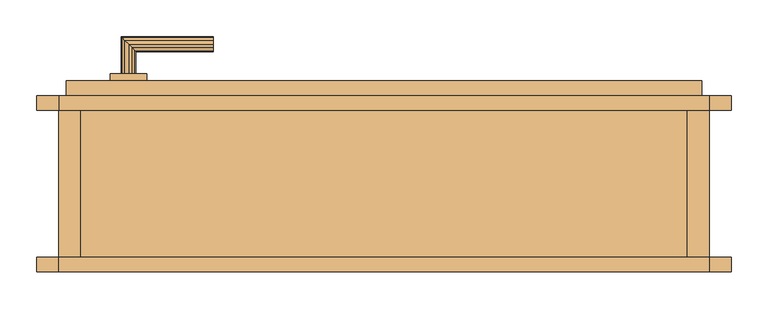
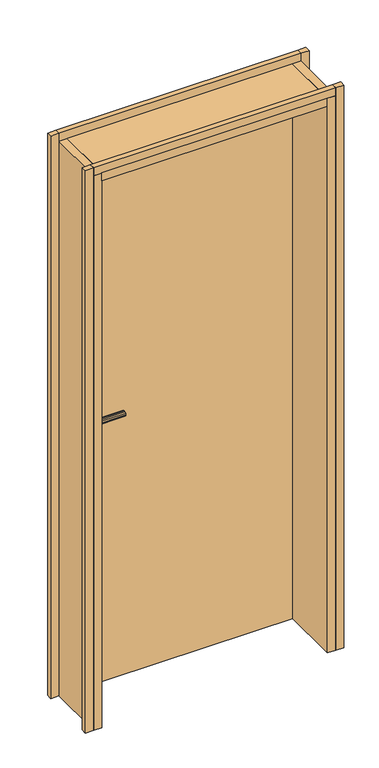
"""IFC4 building model written with IfcOpenShell, lengths in millimetres: door geometry, Tür."""

import ifcopenshell
import ifcopenshell.guid

model = None  # the IFC model being written
_history = None  # IfcOwnerHistory: only IFC2X3 demands one
_inside = {}  # id of a spatial element -> (the spatial element, [elements in it])
_under = {}  # id of a project, library or spatial element -> (it, [spatial elements below it])
_declared = {}  # id of a project -> (the project, [libraries it declares])
_typed = {}  # id of a type object -> (the type object, [elements of that type])
_made_of = {}  # id of a material, layer set ... -> (it, [elements and type objects made of it])


def new_model(schema):
    """Start an empty IFC model of exactly this schema.

    Asked for "IFC4X3", IfcOpenShell would pick the latest addendum, in which some entities
    have other attributes; the version numbers below select the first issue.
    IFC2X3 requires an IfcOwnerHistory on every rooted entity: one is made here for all.
    """
    global model, _history
    if schema == "IFC4X3":
        model = ifcopenshell.file(schema_version=(4, 3, 0, 0))
    else:
        model = ifcopenshell.file(schema=schema)
    _inside.clear()
    _under.clear()
    _declared.clear()
    _typed.clear()
    _made_of.clear()
    _history = None
    if model.schema == "IFC2X3":
        org = make("IfcOrganization", Name="unknown")
        user = make(
            "IfcPersonAndOrganization",
            ThePerson=make("IfcPerson", FamilyName="unknown"),
            TheOrganization=org,
        )
        app = make(
            "IfcApplication",
            ApplicationDeveloper=org,
            Version="unknown",
            ApplicationFullName="unknown",
            ApplicationIdentifier="unknown",
        )
        _history = make(
            "IfcOwnerHistory",
            OwningUser=user,
            OwningApplication=app,
            ChangeAction="ADDED",
            CreationDate=0,
        )
    return model


def make(cls, **values):
    """One entity of the class cls with the attributes given. An attribute that is None is left unset."""
    return model.create_entity(
        cls, **{name: value for name, value in values.items() if value is not None}
    )


def rooted(cls, **values):
    """An entity with a GlobalId (a new one), such as an element, a storey or a relation."""
    return make(cls, GlobalId=ifcopenshell.guid.new(), OwnerHistory=_history, **values)


def si_unit(unit_type, name, prefix=None):
    """IfcSIUnit, for example si_unit("LENGTHUNIT", "METRE", prefix="MILLI")."""
    return make("IfcSIUnit", UnitType=unit_type, Prefix=prefix, Name=name)


def assignment(units):
    """IfcUnitAssignment: the units of a project."""
    return None if units is None else make("IfcUnitAssignment", Units=units)


def point(xyz):
    """IfcCartesianPoint."""
    return None if xyz is None else make("IfcCartesianPoint", Coordinates=xyz)


def direction(xyz):
    """IfcDirection."""
    return None if xyz is None else make("IfcDirection", DirectionRatios=xyz)


def frame(location, z_axis=None, x_axis=None):
    """IfcAxis2Placement3D, a coordinate frame: its origin and axes. An axis left out is left unset."""
    return make(
        "IfcAxis2Placement3D",
        Location=point(location),
        Axis=direction(z_axis),
        RefDirection=direction(x_axis),
    )


def origin():
    """The frame at (0, 0, 0) with its axes left unset."""
    return frame((0.0, 0.0, 0.0))


def place(relative_to, where):
    """IfcLocalPlacement: puts the frame where relative to a parent placement (None: the world)."""
    return make(
        "IfcLocalPlacement", PlacementRelTo=relative_to, RelativePlacement=where
    )


def context(
    kind, dimensions, precision=None, world=None, true_north=None, identifier=None
):
    """IfcGeometricRepresentationContext, for example the 3D "Model" context."""
    return make(
        "IfcGeometricRepresentationContext",
        ContextIdentifier=identifier,
        ContextType=kind,
        CoordinateSpaceDimension=dimensions,
        Precision=precision,
        WorldCoordinateSystem=world,
        TrueNorth=true_north,
    )


def project(units=None, contexts=None):
    """IfcProject with its units and contexts."""
    return rooted(
        "IfcProject",
        Name="project",
        RepresentationContexts=contexts,
        UnitsInContext=assignment(units),
    )


def spatial(cls, under=None, at=None, **own):
    """A site, building, storey or space (cls), placed at a placement, below another one or the project."""
    s = rooted(cls, ObjectPlacement=at, **own)
    if under is not None:
        _under.setdefault(under.id(), (under, []))[1].append(s)
    return s


def polyline(points):
    """IfcPolyline through the points."""
    return make("IfcPolyline", Points=[point(p) for p in points])


def outline(outer, holes=None, kind="AREA"):
    """IfcArbitraryClosedProfileDef: a profile drawn as a closed curve; with holes, ...WithVoids."""
    if holes is None:
        return make("IfcArbitraryClosedProfileDef", ProfileType=kind, OuterCurve=outer)
    return make(
        "IfcArbitraryProfileDefWithVoids",
        ProfileType=kind,
        OuterCurve=outer,
        InnerCurves=holes,
    )


def extrude(swept, where, along, depth):
    """IfcExtrudedAreaSolid: the profile swept, set in the frame where, extruded along a direction by depth."""
    return make(
        "IfcExtrudedAreaSolid",
        SweptArea=swept,
        Position=where,
        ExtrudedDirection=direction(along),
        Depth=depth,
    )


def faces_of(points, faces, orient=None, outer=None):
    """IfcFace entities. A face is a list of loops; a loop is a list of indices into points, from 0.

    orient and outer hold one flag for each loop. By default every Orientation is true, the
    first loop of a face is its IfcFaceOuterBound and the others are IfcFaceBound.
    """
    made = []
    for i, loops in enumerate(faces):
        bounds = []
        for j, loop in enumerate(loops):
            is_outer = j == 0 if outer is None else outer[i][j]
            bounds.append(
                make(
                    "IfcFaceOuterBound" if is_outer else "IfcFaceBound",
                    Bound=make("IfcPolyLoop", Polygon=[points[k] for k in loop]),
                    Orientation=True if orient is None else orient[i][j],
                )
            )
        made.append(make("IfcFace", Bounds=bounds))
    return made


def faceted_brep(points, faces, orient=None, outer=None, voids=None):
    """IfcFacetedBrep: a solid bounded by flat faces; with voids (closed shells), ...WithVoids."""
    shared = [point(p) for p in points]
    hull = make("IfcClosedShell", CfsFaces=faces_of(shared, faces, orient, outer))
    if voids is None:
        return make("IfcFacetedBrep", Outer=hull)
    return make(
        "IfcFacetedBrepWithVoids",
        Outer=hull,
        Voids=[
            make(cls, CfsFaces=faces_of(shared, fs, o, b)) for cls, fs, o, b in voids
        ],
    )


def shape(context_of_items, identifier, shape_type, items):
    """IfcShapeRepresentation: the items that make up one representation, for example the "Body"."""
    return make(
        "IfcShapeRepresentation",
        ContextOfItems=context_of_items,
        RepresentationIdentifier=identifier,
        RepresentationType=shape_type,
        Items=items,
    )


def source(mapping_origin, context_of_items, identifier, shape_type, items):
    """IfcRepresentationMap: a shape defined once, which mapped items show again and again."""
    return make(
        "IfcRepresentationMap",
        MappingOrigin=mapping_origin,
        MappedRepresentation=shape(context_of_items, identifier, shape_type, items),
    )


def transform(
    local_origin,
    x_axis=None,
    y_axis=None,
    z_axis=None,
    scale=None,
    scale2=None,
    scale3=None,
    uniform=True,
):
    """IfcCartesianTransformationOperator3D, or its non-uniform kind. x_axis, y_axis, z_axis: its Axis1, 2, 3."""
    if uniform:
        return make(
            "IfcCartesianTransformationOperator3D",
            Axis1=direction(x_axis),
            Axis2=direction(y_axis),
            LocalOrigin=point(local_origin),
            Scale=scale,
            Axis3=direction(z_axis),
        )
    return make(
        "IfcCartesianTransformationOperator3DnonUniform",
        Axis1=direction(x_axis),
        Axis2=direction(y_axis),
        LocalOrigin=point(local_origin),
        Scale=scale,
        Axis3=direction(z_axis),
        Scale2=scale2,
        Scale3=scale3,
    )


def mapped(mapping_source, mapping_target):
    """IfcMappedItem: shows the shape of a source again, moved by a transform."""
    return make(
        "IfcMappedItem", MappingSource=mapping_source, MappingTarget=mapping_target
    )


def made_of(thing, what):
    """Note that an element or type object is made of a material, layer set ...; save() writes the relation."""
    if what is not None:
        _made_of.setdefault(what.id(), (what, []))[1].append(thing)
    return thing


def element(
    cls,
    number,
    at=None,
    inside=None,
    cuts=None,
    type_object=None,
    material=None,
    context=None,
    identifier="Body",
    shape_type=None,
    held_by="IfcProductDefinitionShape",
    body=None,
    shapes=None,
    **own,
):
    """One element of the class cls, such as IfcWall. Its Tag is "e" and its number.

    at: its placement. inside: the storey or other place that contains it. cuts: it is an
    opening in that element (IfcRelVoidsElement). A single representation is given by context,
    identifier, shape_type and body (its items); several are given by shapes. held_by: the class
    of the entity that holds the representations. save() writes the other relations.
    """
    e = rooted(cls, Tag="e%d" % number, ObjectPlacement=at, **own)
    if body is not None:
        shapes = [shape(context, identifier, shape_type, body)]
    if shapes is not None:
        e.Representation = make(held_by, Representations=shapes)
    if inside is not None:
        _inside.setdefault(inside.id(), (inside, []))[1].append(e)
    if cuts is not None:
        rooted(
            "IfcRelVoidsElement", RelatingBuildingElement=cuts, RelatedOpeningElement=e
        )
    if type_object is not None:
        _typed.setdefault(type_object.id(), (type_object, []))[1].append(e)
    return made_of(e, material)


def aggregate(whole, parts):
    """IfcRelAggregates: a whole, such as a stair, and the parts it consists of."""
    return rooted("IfcRelAggregates", RelatingObject=whole, RelatedObjects=parts)


def save(model, path):
    """Write the relations noted so far, then the file.

    IfcRelAggregates (storeys below a building ...), IfcRelContainedInSpatialStructure (elements
    in a storey), IfcRelDefinesByType, IfcRelAssociatesMaterial and IfcRelDeclares: one each for
    every whole, place, type object, material and project.
    """
    for whole, parts in _under.values():
        aggregate(whole, parts)
    for where, things in _inside.values():
        rooted(
            "IfcRelContainedInSpatialStructure",
            RelatedElements=things,
            RelatingStructure=where,
        )
    for kind, things in _typed.values():
        rooted("IfcRelDefinesByType", RelatedObjects=things, RelatingType=kind)
    for what, things in _made_of.values():
        rooted("IfcRelAssociatesMaterial", RelatedObjects=things, RelatingMaterial=what)
    for by, libraries in _declared.values():
        rooted("IfcRelDeclares", RelatingContext=by, RelatedDefinitions=libraries)
    model.write(path)


def door_0659a678(model_context):
    return source(origin(), model_context, "Body", "SolidModel", [
        extrude(outline(polyline([(885.0, -20.0), (855.0, -20.0), (855.0, 220.0), (885.0, 220.0), (885.0, -20.0)])), frame((0.0, 0.0, 140.0), z_axis=(0.0, 0.0, 1.0), x_axis=(1.0, 0.0, 0.0)), (0.0, 0.0, 1.0), 2145.0),
        extrude(outline(polyline([(0.0, 200.0), (-30.0, 200.0), (-30.0, 220.0), (0.0, 220.0), (0.0, 200.0)])), frame((0.0, 0.0, 140.0), z_axis=(0.0, 0.0, 1.0), x_axis=(1.0, 0.0, 0.0)), (0.0, 0.0, 1.0), 2175.0),
        extrude(outline(polyline([(855.0, -20.0), (30.0, -20.0), (30.0, 220.0), (855.0, 220.0), (855.0, -20.0)])), frame((0.0, 0.0, 2255.0), z_axis=(0.0, 0.0, 1.0), x_axis=(1.0, 0.0, 0.0)), (0.0, 0.0, 1.0), 30.0),
        extrude(outline(polyline([(885.0, -20.0), (0.0, -20.0), (0.0, 0.0), (885.0, 0.0), (885.0, -20.0)])), frame((0.0, 0.0, 2285.0), z_axis=(0.0, 0.0, 1.0), x_axis=(1.0, 0.0, 0.0)), (0.0, 0.0, 1.0), 30.0),
        extrude(outline(polyline([(120.0, 240.0), (70.0, 240.0), (70.0, 250.0), (120.0, 250.0), (120.0, 240.0)])), frame((0.0, 0.0, 1050.0), z_axis=(0.0, 0.0, 1.0), x_axis=(1.0, 0.0, 0.0)), (0.0, 0.0, 1.0), 215.0),
        faceted_brep([(100.0, 250.0, 1198.660254), (95.0, 250.0, 1200.0), (90.0, 250.0, 1198.660254), (86.339746, 250.0, 1195.0), (85.0, 250.0, 1190.0), (86.339746, 250.0, 1185.0), (90.0, 250.0, 1181.339746), (95.0, 250.0, 1180.0), (100.0, 250.0, 1181.339746), (103.660254, 250.0, 1185.0), (105.0, 250.0, 1190.0), (103.660254, 250.0, 1195.0), (95.0, 290.0, 1200.0), (90.0, 295.0, 1198.660254), (86.339746, 298.660254, 1195.0), (85.0, 300.0, 1190.0), (86.339746, 298.660254, 1185.0), (90.0, 295.0, 1181.339746), (95.0, 290.0, 1180.0), (100.0, 285.0, 1181.339746), (103.660254, 281.339746, 1185.0), (105.0, 280.0, 1190.0), (103.660254, 281.339746, 1195.0), (100.0, 285.0, 1198.660254), (210.0, 295.0, 1198.660254), (210.0, 290.0, 1200.0), (210.0, 285.0, 1198.660254), (210.0, 281.339746, 1195.0), (210.0, 280.0, 1190.0), (210.0, 281.339746, 1185.0), (210.0, 285.0, 1181.339746), (210.0, 290.0, 1180.0), (210.0, 295.0, 1181.339746), (210.0, 298.660254, 1185.0), (210.0, 300.0, 1190.0), (210.0, 298.660254, 1195.0)], [[[0, 1, 2, 3, 4, 5, 6, 7, 8, 9, 10, 11]], [[2, 1, 12, 13]], [[3, 2, 13, 14]], [[4, 3, 14, 15]], [[5, 4, 15, 16]], [[6, 5, 16, 17]], [[7, 6, 17, 18]], [[8, 7, 18, 19]], [[9, 8, 19, 20]], [[10, 9, 20, 21]], [[11, 10, 21, 22]], [[0, 11, 22, 23]], [[1, 0, 23, 12]], [[24, 25, 26, 27, 28, 29, 30, 31, 32, 33, 34, 35]], [[13, 12, 25, 24]], [[14, 13, 24, 35]], [[15, 14, 35, 34]], [[16, 15, 34, 33]], [[17, 16, 33, 32]], [[18, 17, 32, 31]], [[19, 18, 31, 30]], [[20, 19, 30, 29]], [[21, 20, 29, 28]], [[22, 21, 28, 27]], [[23, 22, 27, 26]], [[12, 23, 26, 25]]]),
        faceted_brep([(90.0, 190.0, 1198.660254), (95.0, 190.0, 1200.0), (100.0, 190.0, 1198.660254), (103.660254, 190.0, 1195.0), (105.0, 190.0, 1190.0), (103.660254, 190.0, 1185.0), (100.0, 190.0, 1181.339746), (95.0, 190.0, 1180.0), (90.0, 190.0, 1181.339746), (86.339746, 190.0, 1185.0), (85.0, 190.0, 1190.0), (86.339746, 190.0, 1195.0), (95.0, 150.0, 1200.0), (90.0, 145.0, 1198.660254), (86.339746, 141.339746, 1195.0), (85.0, 140.0, 1190.0), (86.339746, 141.339746, 1185.0), (90.0, 145.0, 1181.339746), (95.0, 150.0, 1180.0), (100.0, 155.0, 1181.339746), (103.660254, 158.660254, 1185.0), (105.0, 160.0, 1190.0), (103.660254, 158.660254, 1195.0), (100.0, 155.0, 1198.660254), (210.0, 155.0, 1198.660254), (210.0, 150.0, 1200.0), (210.0, 145.0, 1198.660254), (210.0, 141.339746, 1195.0), (210.0, 140.0, 1190.0), (210.0, 141.339746, 1185.0), (210.0, 145.0, 1181.339746), (210.0, 150.0, 1180.0), (210.0, 155.0, 1181.339746), (210.0, 158.660254, 1185.0), (210.0, 160.0, 1190.0), (210.0, 158.660254, 1195.0)], [[[0, 1, 2, 3, 4, 5, 6, 7, 8, 9, 10, 11]], [[12, 1, 0, 13]], [[13, 0, 11, 14]], [[14, 11, 10, 15]], [[15, 10, 9, 16]], [[16, 9, 8, 17]], [[17, 8, 7, 18]], [[18, 7, 6, 19]], [[19, 6, 5, 20]], [[20, 5, 4, 21]], [[21, 4, 3, 22]], [[22, 3, 2, 23]], [[23, 2, 1, 12]], [[24, 25, 26, 27, 28, 29, 30, 31, 32, 33, 34, 35]], [[25, 12, 13, 26]], [[26, 13, 14, 27]], [[27, 14, 15, 28]], [[28, 15, 16, 29]], [[29, 16, 17, 30]], [[30, 17, 18, 31]], [[31, 18, 19, 32]], [[32, 19, 20, 33]], [[33, 20, 21, 34]], [[34, 21, 22, 35]], [[35, 22, 23, 24]], [[24, 23, 12, 25]]]),
        extrude(outline(polyline([(70.0, 190.0), (70.0, 200.0), (120.0, 200.0), (120.0, 190.0), (70.0, 190.0)])), frame((0.0, 0.0, 1050.0), z_axis=(0.0, 0.0, 1.0), x_axis=(1.0, 0.0, 0.0)), (0.0, 0.0, 1.0), 215.0),
        extrude(outline(polyline([(875.0, 200.0), (10.0, 200.0), (10.0, 240.0), (875.0, 240.0), (875.0, 200.0)])), frame((0.0, 0.0, 140.0), z_axis=(0.0, 0.0, 1.0), x_axis=(1.0, 0.0, 0.0)), (0.0, 0.0, 1.0), 2135.0),
        extrude(outline(polyline([(915.0, 0.0), (915.0, -20.0), (885.0, -20.0), (885.0, 0.0), (915.0, 0.0)])), frame((0.0, 0.0, 140.0), z_axis=(0.0, 0.0, 1.0), x_axis=(1.0, 0.0, 0.0)), (0.0, 0.0, 1.0), 2175.0),
        extrude(outline(polyline([(0.0, -20.0), (-30.0, -20.0), (-30.0, 0.0), (0.0, 0.0), (0.0, -20.0)])), frame((0.0, 0.0, 140.0), z_axis=(0.0, 0.0, 1.0), x_axis=(1.0, 0.0, 0.0)), (0.0, 0.0, 1.0), 2175.0),
        extrude(outline(polyline([(885.0, 200.0), (0.0, 200.0), (0.0, 220.0), (885.0, 220.0), (885.0, 200.0)])), frame((0.0, 0.0, 2285.0), z_axis=(0.0, 0.0, 1.0), x_axis=(1.0, 0.0, 0.0)), (0.0, 0.0, 1.0), 30.0),
        extrude(outline(polyline([(30.0, -20.0), (0.0, -20.0), (0.0, 220.0), (30.0, 220.0), (30.0, -20.0)])), frame((0.0, 0.0, 140.0), z_axis=(0.0, 0.0, 1.0), x_axis=(1.0, 0.0, 0.0)), (0.0, 0.0, 1.0), 2145.0),
        extrude(outline(polyline([(915.0, 220.0), (915.0, 200.0), (885.0, 200.0), (885.0, 220.0), (915.0, 220.0)])), frame((0.0, 0.0, 140.0), z_axis=(0.0, 0.0, 1.0), x_axis=(1.0, 0.0, 0.0)), (0.0, 0.0, 1.0), 2175.0),
    ])


if __name__ == "__main__":
    model = new_model("IFC4")
    model_context = context("Model", 3, world=origin())
    ifc_project = project(units=[si_unit("LENGTHUNIT", "METRE", prefix="MILLI")], contexts=[model_context])
    site = spatial("IfcSite", under=ifc_project)
    building = spatial("IfcBuilding", under=site)
    placement = place(None, origin())
    door_shape = door_0659a678(model_context)
    element("IfcDoor", 1, ObjectType="Tür", at=placement, inside=building, context=model_context, shape_type="MappedRepresentation", body=[
        mapped(door_shape, transform((0.0, 0.0, 0.0), x_axis=(1.0, 0.0, 0.0), y_axis=(0.0, 1.0, 0.0), z_axis=(0.0, 0.0, 1.0))),
    ])
    save(model, "model.ifc")

# Revit data of these elements
# Type "Tür"
#   Type Mark = "38"
# Element 1 (IfcDoor, "Tür")
#   Materials on its faces: "tuer_beschlag", "tuer_holzzarge"
# Materials
#   "tuer_beschlag": class "Unassigned", colour RGB 128 128 128, transparency 0
#   "tuer_holzzarge": class "Unassigned", colour RGB 255 255 255, transparency 0
